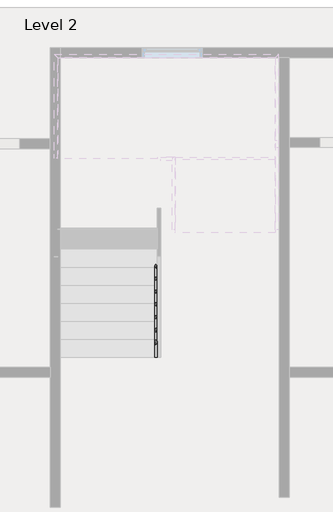
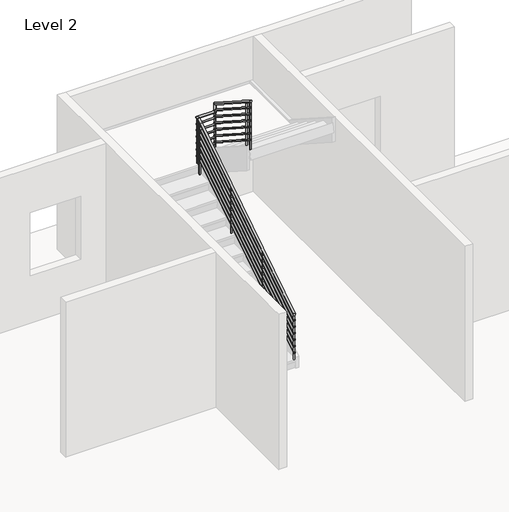
# One storey, part 6 of 7: 1 railing.
"""IFC4 building model written with IfcOpenShell, lengths in millimetres."""

from ifc_helpers import new_model, si_unit, point, frame, frame_2d, origin, place, context, project, spatial, circle_curve, ellipse_curve, trimmed, segment, composite_curve, outline, extrude, element, save
from ifc_brep_helpers import plane_surface, cylinder_surface, advanced_brep

model = new_model("IFC4")

# Units and contexts
model_context = context("Model", 3, world=origin())
ifc_project = project(units=[si_unit("LENGTHUNIT", "METRE", prefix="MILLI")], contexts=[model_context])

# Site, building, storey
site = spatial("IfcSite", under=ifc_project)
building = spatial("IfcBuilding", under=site)
storey = spatial("IfcBuildingStorey", under=building, Name="Level 2", Elevation=3500.0)

# Railing
placement = place(None, origin())
element("IfcRailing", 1, ObjectType="900mm Pipe", at=placement, inside=storey, context=model_context, shape_type="SolidModel", body=[
    advanced_brep(
    [(-504.8393676, 4284.7509075, 4552.7068065), (-544.8393676, 4284.7509075, 4552.7068065), (-504.8393676, 7315.616134, 6497.6470588), (-544.8393676, 7315.616134, 6497.6470588), (-504.8393676, 7337.8781803, 6497.6470588), (-544.8393676, 7377.8781803, 6497.6470588), (-201.3120949, 7337.8781803, 6497.6470588), (-201.3120949, 7377.8781803, 6497.6470588)],
    [
        (0, 1, ellipse_curve(frame((-524.8393676, 4284.7509075, 4552.7068065), z_axis=(0.0, -1.0, 0.0), x_axis=(0.0, 0.0, -1.0)), 23.7637817, 20.0)),
        (1, 0, ellipse_curve(frame((-524.8393676, 4284.7509075, 4552.7068065), z_axis=(0.0, -1.0, 0.0), x_axis=(0.0, 0.0, -1.0)), 23.7637817, 20.0)),
        (0, 2),
        (2, 3, ellipse_curve(frame((-524.8393676, 7315.616134, 6497.6470588), z_axis=(0.0, -0.9595876426002529, -0.2814099432658509), x_axis=(0.0, 0.2814099432658507, -0.9595876426002528)), 20.8422859, 20.0)),
        (3, 1),
        (3, 2, ellipse_curve(frame((-524.8393676, 7315.616134, 6497.6470588), z_axis=(0.0, -0.9595876426002529, -0.2814099432658509), x_axis=(0.0, 0.2814099432658507, -0.9595876426002528)), 20.8422859, 20.0)),
        (2, 4),
        (4, 5, ellipse_curve(frame((-524.8393676, 7357.8781803, 6497.6470588), z_axis=(-0.7071067811865475, -0.7071067811865475, 0.0), x_axis=(0.7071067811865474, -0.7071067811865476, 0.0)), 28.2842712, 20.0)),
        (5, 3),
        (5, 4, ellipse_curve(frame((-524.8393676, 7357.8781803, 6497.6470588), z_axis=(-0.7071067811865475, -0.7071067811865475, 0.0), x_axis=(0.7071067811865474, -0.7071067811865476, 0.0)), 28.2842712, 20.0)),
        (6, 7, ellipse_curve(frame((-201.3120949, 7357.8781803, 6497.6470588), z_axis=(0.7071067811865476, 0.0, 0.7071067811865476), x_axis=(-0.7071067811865474, 0.0, 0.7071067811865476)), 28.2842712, 20.0)),
        (7, 6, ellipse_curve(frame((-201.3120949, 7357.8781803, 6497.6470588), z_axis=(0.7071067811865476, 0.0, 0.7071067811865476), x_axis=(-0.7071067811865474, 0.0, 0.7071067811865476)), 28.2842712, 20.0)),
        (4, 6),
        (7, 5),
    ],
    [
        plane_surface(frame((-524.8393676, 4284.7509075, 4576.4705882), z_axis=(0.0, -1.0, 0.0), x_axis=(0.0, 0.0, 1.0))),
        cylinder_surface(frame((-524.8393676, 4295.5524077, 4559.6382505), z_axis=(0.0, -0.8416168876622212, -0.5400750081254976), x_axis=(-1.0, 0.0, 0.0)), 20.0),
        cylinder_surface(frame((-524.8393676, 7309.7509075, 6497.6470588), z_axis=(0.0, -1.0, 0.0), x_axis=(-1.0, 0.0, 0.0)), 20.0),
        plane_surface(frame((-221.3120949, 7357.8781803, 6517.6470588), z_axis=(0.7071067811865476, 0.0, 0.7071067811865476), x_axis=(0.7071067811865476, 0.0, -0.7071067811865476))),
        cylinder_surface(frame((-524.8393676, 7357.8781803, 6497.6470588), z_axis=(-1.0, 0.0, 0.0), x_axis=(0.0, 1.0, 0.0)), 20.0),
    ],
    [
        (0, [[1, 2]]),
        (1, [[-1, 3, 4, 5]]),
        (1, [[-2, -5, 6, -3]]),
        (2, [[-4, 7, 8, 9]]),
        (2, [[-6, -9, 10, -7]]),
        (3, [[11, 12]]),
        (4, [[-8, 13, -12, 14]]),
        (4, [[-10, -14, -11, -13]]),
    ],
),
    advanced_brep(
    [(-201.3120949, 7337.8781803, 6497.6470588), (-201.3120949, 7377.8781803, 6497.6470588), (-201.3120949, 7337.8781803, 6643.124843), (-201.3120949, 7377.8781803, 6664.9839572)],
    [
        (0, 1, ellipse_curve(frame((-201.3120949, 7357.8781803, 6497.6470588), z_axis=(-0.7071067811865476, 0.0, -0.7071067811865476), x_axis=(0.7071067811865476, 0.0, -0.7071067811865474)), 28.2842712, 20.0)),
        (1, 0, ellipse_curve(frame((-201.3120949, 7357.8781803, 6497.6470588), z_axis=(-0.7071067811865476, 0.0, -0.7071067811865476), x_axis=(0.7071067811865476, 0.0, -0.7071067811865474)), 28.2842712, 20.0)),
        (2, 3, ellipse_curve(frame((-201.3120949, 7357.8781803, 6654.0544001), z_axis=(0.0, -0.47954405004884676, 0.877517808402057), x_axis=(0.0, -0.8775178084020571, -0.47954405004884676)), 22.7915602, 20.0)),
        (3, 2, ellipse_curve(frame((-201.3120949, 7357.8781803, 6654.0544001), z_axis=(0.0, -0.47954405004884676, 0.877517808402057), x_axis=(0.0, -0.8775178084020571, -0.47954405004884676)), 22.7915602, 20.0)),
        (0, 2),
        (3, 1),
    ],
    [
        plane_surface(frame((-201.3120949, 7357.8781803, 6497.6470588), z_axis=(-0.7071067811865476, 0.0, -0.7071067811865476), x_axis=(0.7071067811865476, 0.0, -0.7071067811865476))),
        plane_surface(frame((-201.3120949, 7357.8781803, 6654.0544001), z_axis=(0.0, -0.47954405004884676, 0.877517808402057), x_axis=(1.0, 0.0, 0.0))),
        cylinder_surface(frame((-201.3120949, 7357.8781803, 6497.6470588), z_axis=(0.0, 0.0, -1.0), x_axis=(0.0, 1.0, 0.0)), 20.0),
    ],
    [
        (0, [[1, 2]]),
        (1, [[3, 4]]),
        (2, [[-1, 5, -4, 6]]),
        (2, [[-2, -6, -3, -5]]),
    ],
),
    advanced_brep(
    [(-221.3120949, 7357.8781803, 6654.0544001), (-181.3120949, 7357.8781803, 6654.0544001), (-221.3120949, 6232.4781803, 7376.2362183), (-181.3120949, 6232.4781803, 7376.2362183)],
    [
        (0, 1, ellipse_curve(frame((-201.3120949, 7357.8781803, 6654.0544001), z_axis=(0.0, 0.47954405004884676, -0.877517808402057), x_axis=(0.0, 0.8775178084020568, 0.47954405004884676)), 22.7915602, 20.0)),
        (1, 0, ellipse_curve(frame((-201.3120949, 7357.8781803, 6654.0544001), z_axis=(0.0, 0.47954405004884676, -0.877517808402057), x_axis=(0.0, 0.8775178084020568, 0.47954405004884676)), 22.7915602, 20.0)),
        (2, 3, ellipse_curve(frame((-201.3120949, 6232.4781803, 7376.2362183), z_axis=(0.0, -1.0, 0.0), x_axis=(0.0, 0.0, -1.0)), 23.7637817, 20.0)),
        (3, 2, ellipse_curve(frame((-201.3120949, 6232.4781803, 7376.2362183), z_axis=(0.0, -1.0, 0.0), x_axis=(0.0, 0.0, -1.0)), 23.7637817, 20.0)),
        (0, 2),
        (3, 1),
    ],
    [
        plane_surface(frame((-201.3120949, 7377.8781803, 6664.9839572), z_axis=(0.0, 0.47954405004884676, -0.877517808402057), x_axis=(1.0, 0.0, 0.0))),
        plane_surface(frame((-201.3120949, 6232.4781803, 7400.0), z_axis=(0.0, -1.0, 0.0), x_axis=(0.0, 0.0, -1.0))),
        cylinder_surface(frame((-201.3120949, 7367.0766801, 6648.1516195), z_axis=(0.0, 0.8416168876622208, -0.5400750081254984), x_axis=(1.0, 0.0, 0.0)), 20.0),
    ],
    [
        (0, [[1, 2]]),
        (1, [[3, 4]]),
        (2, [[-1, 5, -4, 6]]),
        (2, [[-2, -6, -3, -5]]),
    ],
),
    advanced_brep(
    [(-539.8393676, 4284.7509075, 4433.647752), (-509.8393676, 4284.7509075, 4433.647752), (-539.8393676, 7309.7509075, 6374.8242225), (-509.8393676, 7309.7509075, 6374.8242225)],
    [
        (0, 1, ellipse_curve(frame((-524.8393676, 4284.7509075, 4433.647752), z_axis=(0.0, -1.0, 0.0), x_axis=(0.0, 0.0, -1.0)), 17.8228363, 15.0)),
        (1, 0, ellipse_curve(frame((-524.8393676, 4284.7509075, 4433.647752), z_axis=(0.0, -1.0, 0.0), x_axis=(0.0, 0.0, -1.0)), 17.8228363, 15.0)),
        (2, 3, ellipse_curve(frame((-524.8393676, 7309.7509075, 6374.8242225), z_axis=(0.0, 1.0, 0.0), x_axis=(0.0, 0.0, -1.0)), 17.8228363, 15.0)),
        (3, 2, ellipse_curve(frame((-524.8393676, 7309.7509075, 6374.8242225), z_axis=(0.0, 1.0, 0.0), x_axis=(0.0, 0.0, -1.0)), 17.8228363, 15.0)),
        (0, 2),
        (3, 1),
    ],
    [
        plane_surface(frame((-524.8393676, 4284.7509075, 4451.4705882), z_axis=(0.0, -1.0, 0.0), x_axis=(0.0, 0.0, 1.0))),
        plane_surface(frame((-524.8393676, 7309.7509075, 6392.6470588), z_axis=(0.0, 1.0, 0.0), x_axis=(0.0, 0.0, 1.0))),
        cylinder_surface(frame((-524.8393676, 4292.8520327, 4438.8463349), z_axis=(0.0, -0.8416168876622212, -0.5400750081254976), x_axis=(1.0, 0.0, 0.0)), 15.0),
    ],
    [
        (0, [[1, 2]]),
        (1, [[3, 4]]),
        (2, [[-1, 5, -4, 6]]),
        (2, [[-2, -6, -3, -5]]),
    ],
),
    advanced_brep(
    [(-539.8393676, 7309.7509075, 6377.6470588), (-509.8393676, 7309.7509075, 6377.6470588), (-539.8393676, 7342.8781803, 6377.6470588), (-509.8393676, 7342.8781803, 6377.6470588)],
    [
        (0, 1, circle_curve(frame((-524.8393676, 7309.7509075, 6377.6470588), z_axis=(0.0, -1.0, 0.0), x_axis=(1.0, 0.0, 0.0)), 15.0)),
        (1, 0, circle_curve(frame((-524.8393676, 7309.7509075, 6377.6470588), z_axis=(0.0, -1.0, 0.0), x_axis=(1.0, 0.0, 0.0)), 15.0)),
        (2, 3, circle_curve(frame((-524.8393676, 7342.8781803, 6377.6470588), z_axis=(0.0, 1.0, 0.0), x_axis=(1.0, 0.0, 0.0)), 15.0)),
        (3, 2, circle_curve(frame((-524.8393676, 7342.8781803, 6377.6470588), z_axis=(0.0, 1.0, 0.0), x_axis=(1.0, 0.0, 0.0)), 15.0)),
        (0, 2),
        (3, 1),
    ],
    [
        plane_surface(frame((-524.8393676, 7309.7509075, 6392.6470588), z_axis=(0.0, -1.0, 0.0), x_axis=(0.0, 0.0, 1.0))),
        plane_surface(frame((-524.8393676, 7342.8781803, 6392.6470588), z_axis=(0.0, 1.0, 0.0), x_axis=(0.0, 0.0, 1.0))),
        cylinder_surface(frame((-524.8393676, 7309.7509075, 6377.6470588), z_axis=(0.0, -1.0, 0.0), x_axis=(1.0, 0.0, 0.0)), 15.0),
    ],
    [
        (0, [[1, 2]]),
        (1, [[3, 4]]),
        (2, [[-1, 5, -4, 6]]),
        (2, [[-2, -6, -3, -5]]),
    ],
),
    advanced_brep(
    [(-539.8393676, 7372.8781803, 6377.6470588), (-539.8393676, 7342.8781803, 6377.6470588), (-216.3120949, 7372.8781803, 6377.6470588), (-216.3120949, 7342.8781803, 6377.6470588)],
    [
        (0, 1, circle_curve(frame((-539.8393676, 7357.8781803, 6377.6470588), z_axis=(-1.0, 0.0, 0.0), x_axis=(0.0, -1.0, 0.0)), 15.0)),
        (1, 0, circle_curve(frame((-539.8393676, 7357.8781803, 6377.6470588), z_axis=(-1.0, 0.0, 0.0), x_axis=(0.0, -1.0, 0.0)), 15.0)),
        (2, 3, circle_curve(frame((-216.3120949, 7357.8781803, 6377.6470588), z_axis=(1.0, 0.0, 0.0), x_axis=(0.0, -1.0, 0.0)), 15.0)),
        (3, 2, circle_curve(frame((-216.3120949, 7357.8781803, 6377.6470588), z_axis=(1.0, 0.0, 0.0), x_axis=(0.0, -1.0, 0.0)), 15.0)),
        (0, 2),
        (3, 1),
    ],
    [
        plane_surface(frame((-539.8393676, 7357.8781803, 6392.6470588), z_axis=(-1.0, 0.0, 0.0), x_axis=(0.0, 1.0, 0.0))),
        plane_surface(frame((-216.3120949, 7357.8781803, 6392.6470588), z_axis=(1.0, 0.0, 0.0), x_axis=(0.0, 1.0, 0.0))),
        cylinder_surface(frame((-539.8393676, 7357.8781803, 6377.6470588), z_axis=(-1.0, 0.0, 0.0), x_axis=(0.0, -1.0, 0.0)), 15.0),
    ],
    [
        (0, [[1, 2]]),
        (1, [[3, 4]]),
        (2, [[-1, 5, -4, 6]]),
        (2, [[-2, -6, -3, -5]]),
    ],
),
    advanced_brep(
    [(-186.3120949, 7372.8781803, 6525.3696771), (-216.3120949, 7372.8781803, 6525.3696771), (-186.3120949, 6232.4781803, 7257.1771637), (-216.3120949, 6232.4781803, 7257.1771637)],
    [
        (0, 1, ellipse_curve(frame((-201.3120949, 7372.8781803, 6525.3696771), z_axis=(0.0, 1.0, 0.0), x_axis=(0.0, 0.0, -1.0)), 17.8228363, 15.0)),
        (1, 0, ellipse_curve(frame((-201.3120949, 7372.8781803, 6525.3696771), z_axis=(0.0, 1.0, 0.0), x_axis=(0.0, 0.0, -1.0)), 17.8228363, 15.0)),
        (2, 3, ellipse_curve(frame((-201.3120949, 6232.4781803, 7257.1771637), z_axis=(0.0, -1.0, 0.0), x_axis=(0.0, 0.0, -1.0)), 17.8228363, 15.0)),
        (3, 2, ellipse_curve(frame((-201.3120949, 6232.4781803, 7257.1771637), z_axis=(0.0, -1.0, 0.0), x_axis=(0.0, 0.0, -1.0)), 17.8228363, 15.0)),
        (0, 2),
        (3, 1),
    ],
    [
        plane_surface(frame((-201.3120949, 7372.8781803, 6543.1925134), z_axis=(0.0, 1.0, 0.0), x_axis=(0.0, 0.0, -1.0))),
        plane_surface(frame((-201.3120949, 6232.4781803, 7275.0), z_axis=(0.0, -1.0, 0.0), x_axis=(0.0, 0.0, -1.0))),
        cylinder_surface(frame((-201.3120949, 7364.7770552, 6530.5682601), z_axis=(0.0, 0.8416168876622208, -0.5400750081254984), x_axis=(-1.0, 0.0, 0.0)), 15.0),
    ],
    [
        (0, [[1, 2]]),
        (1, [[3, 4]]),
        (2, [[-1, 5, -4, 6]]),
        (2, [[-2, -6, -3, -5]]),
    ],
),
    advanced_brep(
    [(-539.8393676, 4284.7509075, 4308.647752), (-509.8393676, 4284.7509075, 4308.647752), (-539.8393676, 7309.7509075, 6249.8242225), (-509.8393676, 7309.7509075, 6249.8242225)],
    [
        (0, 1, ellipse_curve(frame((-524.8393676, 4284.7509075, 4308.647752), z_axis=(0.0, -1.0, 0.0), x_axis=(0.0, 0.0, -1.0)), 17.8228363, 15.0)),
        (1, 0, ellipse_curve(frame((-524.8393676, 4284.7509075, 4308.647752), z_axis=(0.0, -1.0, 0.0), x_axis=(0.0, 0.0, -1.0)), 17.8228363, 15.0)),
        (2, 3, ellipse_curve(frame((-524.8393676, 7309.7509075, 6249.8242225), z_axis=(0.0, 1.0, 0.0), x_axis=(0.0, 0.0, -1.0)), 17.8228363, 15.0)),
        (3, 2, ellipse_curve(frame((-524.8393676, 7309.7509075, 6249.8242225), z_axis=(0.0, 1.0, 0.0), x_axis=(0.0, 0.0, -1.0)), 17.8228363, 15.0)),
        (0, 2),
        (3, 1),
    ],
    [
        plane_surface(frame((-524.8393676, 4284.7509075, 4326.4705882), z_axis=(0.0, -1.0, 0.0), x_axis=(0.0, 0.0, 1.0))),
        plane_surface(frame((-524.8393676, 7309.7509075, 6267.6470588), z_axis=(0.0, 1.0, 0.0), x_axis=(0.0, 0.0, 1.0))),
        cylinder_surface(frame((-524.8393676, 4292.8520327, 4313.8463349), z_axis=(0.0, -0.8416168876622212, -0.5400750081254976), x_axis=(1.0, 0.0, 0.0)), 15.0),
    ],
    [
        (0, [[1, 2]]),
        (1, [[3, 4]]),
        (2, [[-1, 5, -4, 6]]),
        (2, [[-2, -6, -3, -5]]),
    ],
),
    advanced_brep(
    [(-539.8393676, 7309.7509075, 6252.6470588), (-509.8393676, 7309.7509075, 6252.6470588), (-539.8393676, 7342.8781803, 6252.6470588), (-509.8393676, 7342.8781803, 6252.6470588)],
    [
        (0, 1, circle_curve(frame((-524.8393676, 7309.7509075, 6252.6470588), z_axis=(0.0, -1.0, 0.0), x_axis=(1.0, 0.0, 0.0)), 15.0)),
        (1, 0, circle_curve(frame((-524.8393676, 7309.7509075, 6252.6470588), z_axis=(0.0, -1.0, 0.0), x_axis=(1.0, 0.0, 0.0)), 15.0)),
        (2, 3, circle_curve(frame((-524.8393676, 7342.8781803, 6252.6470588), z_axis=(0.0, 1.0, 0.0), x_axis=(1.0, 0.0, 0.0)), 15.0)),
        (3, 2, circle_curve(frame((-524.8393676, 7342.8781803, 6252.6470588), z_axis=(0.0, 1.0, 0.0), x_axis=(1.0, 0.0, 0.0)), 15.0)),
        (0, 2),
        (3, 1),
    ],
    [
        plane_surface(frame((-524.8393676, 7309.7509075, 6267.6470588), z_axis=(0.0, -1.0, 0.0), x_axis=(0.0, 0.0, 1.0))),
        plane_surface(frame((-524.8393676, 7342.8781803, 6267.6470588), z_axis=(0.0, 1.0, 0.0), x_axis=(0.0, 0.0, 1.0))),
        cylinder_surface(frame((-524.8393676, 7309.7509075, 6252.6470588), z_axis=(0.0, -1.0, 0.0), x_axis=(1.0, 0.0, 0.0)), 15.0),
    ],
    [
        (0, [[1, 2]]),
        (1, [[3, 4]]),
        (2, [[-1, 5, -4, 6]]),
        (2, [[-2, -6, -3, -5]]),
    ],
),
    advanced_brep(
    [(-539.8393676, 7372.8781803, 6252.6470588), (-539.8393676, 7342.8781803, 6252.6470588), (-216.3120949, 7372.8781803, 6252.6470588), (-216.3120949, 7342.8781803, 6252.6470588)],
    [
        (0, 1, circle_curve(frame((-539.8393676, 7357.8781803, 6252.6470588), z_axis=(-1.0, 0.0, 0.0), x_axis=(0.0, -1.0, 0.0)), 15.0)),
        (1, 0, circle_curve(frame((-539.8393676, 7357.8781803, 6252.6470588), z_axis=(-1.0, 0.0, 0.0), x_axis=(0.0, -1.0, 0.0)), 15.0)),
        (2, 3, circle_curve(frame((-216.3120949, 7357.8781803, 6252.6470588), z_axis=(1.0, 0.0, 0.0), x_axis=(0.0, -1.0, 0.0)), 15.0)),
        (3, 2, circle_curve(frame((-216.3120949, 7357.8781803, 6252.6470588), z_axis=(1.0, 0.0, 0.0), x_axis=(0.0, -1.0, 0.0)), 15.0)),
        (0, 2),
        (3, 1),
    ],
    [
        plane_surface(frame((-539.8393676, 7357.8781803, 6267.6470588), z_axis=(-1.0, 0.0, 0.0), x_axis=(0.0, 1.0, 0.0))),
        plane_surface(frame((-216.3120949, 7357.8781803, 6267.6470588), z_axis=(1.0, 0.0, 0.0), x_axis=(0.0, 1.0, 0.0))),
        cylinder_surface(frame((-539.8393676, 7357.8781803, 6252.6470588), z_axis=(-1.0, 0.0, 0.0), x_axis=(0.0, -1.0, 0.0)), 15.0),
    ],
    [
        (0, [[1, 2]]),
        (1, [[3, 4]]),
        (2, [[-1, 5, -4, 6]]),
        (2, [[-2, -6, -3, -5]]),
    ],
),
    advanced_brep(
    [(-186.3120949, 7372.8781803, 6400.3696771), (-216.3120949, 7372.8781803, 6400.3696771), (-186.3120949, 6232.4781803, 7132.1771637), (-216.3120949, 6232.4781803, 7132.1771637)],
    [
        (0, 1, ellipse_curve(frame((-201.3120949, 7372.8781803, 6400.3696771), z_axis=(0.0, 1.0, 0.0), x_axis=(0.0, 0.0, -1.0)), 17.8228363, 15.0)),
        (1, 0, ellipse_curve(frame((-201.3120949, 7372.8781803, 6400.3696771), z_axis=(0.0, 1.0, 0.0), x_axis=(0.0, 0.0, -1.0)), 17.8228363, 15.0)),
        (2, 3, ellipse_curve(frame((-201.3120949, 6232.4781803, 7132.1771637), z_axis=(0.0, -1.0, 0.0), x_axis=(0.0, 0.0, -1.0)), 17.8228363, 15.0)),
        (3, 2, ellipse_curve(frame((-201.3120949, 6232.4781803, 7132.1771637), z_axis=(0.0, -1.0, 0.0), x_axis=(0.0, 0.0, -1.0)), 17.8228363, 15.0)),
        (0, 2),
        (3, 1),
    ],
    [
        plane_surface(frame((-201.3120949, 7372.8781803, 6418.1925134), z_axis=(0.0, 1.0, 0.0), x_axis=(0.0, 0.0, -1.0))),
        plane_surface(frame((-201.3120949, 6232.4781803, 7150.0), z_axis=(0.0, -1.0, 0.0), x_axis=(0.0, 0.0, -1.0))),
        cylinder_surface(frame((-201.3120949, 7364.7770552, 6405.5682601), z_axis=(0.0, 0.8416168876622208, -0.5400750081254984), x_axis=(-1.0, 0.0, 0.0)), 15.0),
    ],
    [
        (0, [[1, 2]]),
        (1, [[3, 4]]),
        (2, [[-1, 5, -4, 6]]),
        (2, [[-2, -6, -3, -5]]),
    ],
),
    advanced_brep(
    [(-539.8393676, 4284.7509075, 4183.647752), (-509.8393676, 4284.7509075, 4183.647752), (-539.8393676, 7309.7509075, 6124.8242225), (-509.8393676, 7309.7509075, 6124.8242225)],
    [
        (0, 1, ellipse_curve(frame((-524.8393676, 4284.7509075, 4183.647752), z_axis=(0.0, -1.0, 0.0), x_axis=(0.0, 0.0, -1.0)), 17.8228363, 15.0)),
        (1, 0, ellipse_curve(frame((-524.8393676, 4284.7509075, 4183.647752), z_axis=(0.0, -1.0, 0.0), x_axis=(0.0, 0.0, -1.0)), 17.8228363, 15.0)),
        (2, 3, ellipse_curve(frame((-524.8393676, 7309.7509075, 6124.8242225), z_axis=(0.0, 1.0, 0.0), x_axis=(0.0, 0.0, -1.0)), 17.8228363, 15.0)),
        (3, 2, ellipse_curve(frame((-524.8393676, 7309.7509075, 6124.8242225), z_axis=(0.0, 1.0, 0.0), x_axis=(0.0, 0.0, -1.0)), 17.8228363, 15.0)),
        (0, 2),
        (3, 1),
    ],
    [
        plane_surface(frame((-524.8393676, 4284.7509075, 4201.4705882), z_axis=(0.0, -1.0, 0.0), x_axis=(0.0, 0.0, 1.0))),
        plane_surface(frame((-524.8393676, 7309.7509075, 6142.6470588), z_axis=(0.0, 1.0, 0.0), x_axis=(0.0, 0.0, 1.0))),
        cylinder_surface(frame((-524.8393676, 4292.8520327, 4188.8463349), z_axis=(0.0, -0.8416168876622212, -0.5400750081254976), x_axis=(1.0, 0.0, 0.0)), 15.0),
    ],
    [
        (0, [[1, 2]]),
        (1, [[3, 4]]),
        (2, [[-1, 5, -4, 6]]),
        (2, [[-2, -6, -3, -5]]),
    ],
),
    advanced_brep(
    [(-539.8393676, 7309.7509075, 6127.6470588), (-509.8393676, 7309.7509075, 6127.6470588), (-539.8393676, 7342.8781803, 6127.6470588), (-509.8393676, 7342.8781803, 6127.6470588)],
    [
        (0, 1, circle_curve(frame((-524.8393676, 7309.7509075, 6127.6470588), z_axis=(0.0, -1.0, 0.0), x_axis=(1.0, 0.0, 0.0)), 15.0)),
        (1, 0, circle_curve(frame((-524.8393676, 7309.7509075, 6127.6470588), z_axis=(0.0, -1.0, 0.0), x_axis=(1.0, 0.0, 0.0)), 15.0)),
        (2, 3, circle_curve(frame((-524.8393676, 7342.8781803, 6127.6470588), z_axis=(0.0, 1.0, 0.0), x_axis=(1.0, 0.0, 0.0)), 15.0)),
        (3, 2, circle_curve(frame((-524.8393676, 7342.8781803, 6127.6470588), z_axis=(0.0, 1.0, 0.0), x_axis=(1.0, 0.0, 0.0)), 15.0)),
        (0, 2),
        (3, 1),
    ],
    [
        plane_surface(frame((-524.8393676, 7309.7509075, 6142.6470588), z_axis=(0.0, -1.0, 0.0), x_axis=(0.0, 0.0, 1.0))),
        plane_surface(frame((-524.8393676, 7342.8781803, 6142.6470588), z_axis=(0.0, 1.0, 0.0), x_axis=(0.0, 0.0, 1.0))),
        cylinder_surface(frame((-524.8393676, 7309.7509075, 6127.6470588), z_axis=(0.0, -1.0, 0.0), x_axis=(1.0, 0.0, 0.0)), 15.0),
    ],
    [
        (0, [[1, 2]]),
        (1, [[3, 4]]),
        (2, [[-1, 5, -4, 6]]),
        (2, [[-2, -6, -3, -5]]),
    ],
),
    advanced_brep(
    [(-539.8393676, 7372.8781803, 6127.6470588), (-539.8393676, 7342.8781803, 6127.6470588), (-216.3120949, 7372.8781803, 6127.6470588), (-216.3120949, 7342.8781803, 6127.6470588)],
    [
        (0, 1, circle_curve(frame((-539.8393676, 7357.8781803, 6127.6470588), z_axis=(-1.0, 0.0, 0.0), x_axis=(0.0, -1.0, 0.0)), 15.0)),
        (1, 0, circle_curve(frame((-539.8393676, 7357.8781803, 6127.6470588), z_axis=(-1.0, 0.0, 0.0), x_axis=(0.0, -1.0, 0.0)), 15.0)),
        (2, 3, circle_curve(frame((-216.3120949, 7357.8781803, 6127.6470588), z_axis=(1.0, 0.0, 0.0), x_axis=(0.0, -1.0, 0.0)), 15.0)),
        (3, 2, circle_curve(frame((-216.3120949, 7357.8781803, 6127.6470588), z_axis=(1.0, 0.0, 0.0), x_axis=(0.0, -1.0, 0.0)), 15.0)),
        (0, 2),
        (3, 1),
    ],
    [
        plane_surface(frame((-539.8393676, 7357.8781803, 6142.6470588), z_axis=(-1.0, 0.0, 0.0), x_axis=(0.0, 1.0, 0.0))),
        plane_surface(frame((-216.3120949, 7357.8781803, 6142.6470588), z_axis=(1.0, 0.0, 0.0), x_axis=(0.0, 1.0, 0.0))),
        cylinder_surface(frame((-539.8393676, 7357.8781803, 6127.6470588), z_axis=(-1.0, 0.0, 0.0), x_axis=(0.0, -1.0, 0.0)), 15.0),
    ],
    [
        (0, [[1, 2]]),
        (1, [[3, 4]]),
        (2, [[-1, 5, -4, 6]]),
        (2, [[-2, -6, -3, -5]]),
    ],
),
    advanced_brep(
    [(-186.3120949, 7372.8781803, 6275.3696771), (-216.3120949, 7372.8781803, 6275.3696771), (-186.3120949, 6232.4781803, 7007.1771637), (-216.3120949, 6232.4781803, 7007.1771637)],
    [
        (0, 1, ellipse_curve(frame((-201.3120949, 7372.8781803, 6275.3696771), z_axis=(0.0, 1.0, 0.0), x_axis=(0.0, 0.0, -1.0)), 17.8228363, 15.0)),
        (1, 0, ellipse_curve(frame((-201.3120949, 7372.8781803, 6275.3696771), z_axis=(0.0, 1.0, 0.0), x_axis=(0.0, 0.0, -1.0)), 17.8228363, 15.0)),
        (2, 3, ellipse_curve(frame((-201.3120949, 6232.4781803, 7007.1771637), z_axis=(0.0, -1.0, 0.0), x_axis=(0.0, 0.0, -1.0)), 17.8228363, 15.0)),
        (3, 2, ellipse_curve(frame((-201.3120949, 6232.4781803, 7007.1771637), z_axis=(0.0, -1.0, 0.0), x_axis=(0.0, 0.0, -1.0)), 17.8228363, 15.0)),
        (0, 2),
        (3, 1),
    ],
    [
        plane_surface(frame((-201.3120949, 7372.8781803, 6293.1925134), z_axis=(0.0, 1.0, 0.0), x_axis=(0.0, 0.0, -1.0))),
        plane_surface(frame((-201.3120949, 6232.4781803, 7025.0), z_axis=(0.0, -1.0, 0.0), x_axis=(0.0, 0.0, -1.0))),
        cylinder_surface(frame((-201.3120949, 7364.7770552, 6280.5682601), z_axis=(0.0, 0.8416168876622208, -0.5400750081254984), x_axis=(-1.0, 0.0, 0.0)), 15.0),
    ],
    [
        (0, [[1, 2]]),
        (1, [[3, 4]]),
        (2, [[-1, 5, -4, 6]]),
        (2, [[-2, -6, -3, -5]]),
    ],
),
    advanced_brep(
    [(-539.8393676, 4284.7509075, 4058.647752), (-509.8393676, 4284.7509075, 4058.647752), (-539.8393676, 7309.7509075, 5999.8242225), (-509.8393676, 7309.7509075, 5999.8242225)],
    [
        (0, 1, ellipse_curve(frame((-524.8393676, 4284.7509075, 4058.647752), z_axis=(0.0, -1.0, 0.0), x_axis=(0.0, 0.0, -1.0)), 17.8228363, 15.0)),
        (1, 0, ellipse_curve(frame((-524.8393676, 4284.7509075, 4058.647752), z_axis=(0.0, -1.0, 0.0), x_axis=(0.0, 0.0, -1.0)), 17.8228363, 15.0)),
        (2, 3, ellipse_curve(frame((-524.8393676, 7309.7509075, 5999.8242225), z_axis=(0.0, 1.0, 0.0), x_axis=(0.0, 0.0, -1.0)), 17.8228363, 15.0)),
        (3, 2, ellipse_curve(frame((-524.8393676, 7309.7509075, 5999.8242225), z_axis=(0.0, 1.0, 0.0), x_axis=(0.0, 0.0, -1.0)), 17.8228363, 15.0)),
        (0, 2),
        (3, 1),
    ],
    [
        plane_surface(frame((-524.8393676, 4284.7509075, 4076.4705882), z_axis=(0.0, -1.0, 0.0), x_axis=(0.0, 0.0, 1.0))),
        plane_surface(frame((-524.8393676, 7309.7509075, 6017.6470588), z_axis=(0.0, 1.0, 0.0), x_axis=(0.0, 0.0, 1.0))),
        cylinder_surface(frame((-524.8393676, 4292.8520327, 4063.8463349), z_axis=(0.0, -0.8416168876622212, -0.5400750081254976), x_axis=(1.0, 0.0, 0.0)), 15.0),
    ],
    [
        (0, [[1, 2]]),
        (1, [[3, 4]]),
        (2, [[-1, 5, -4, 6]]),
        (2, [[-2, -6, -3, -5]]),
    ],
),
    advanced_brep(
    [(-539.8393676, 7309.7509075, 6002.6470588), (-509.8393676, 7309.7509075, 6002.6470588), (-539.8393676, 7342.8781803, 6002.6470588), (-509.8393676, 7342.8781803, 6002.6470588)],
    [
        (0, 1, circle_curve(frame((-524.8393676, 7309.7509075, 6002.6470588), z_axis=(0.0, -1.0, 0.0), x_axis=(1.0, 0.0, 0.0)), 15.0)),
        (1, 0, circle_curve(frame((-524.8393676, 7309.7509075, 6002.6470588), z_axis=(0.0, -1.0, 0.0), x_axis=(1.0, 0.0, 0.0)), 15.0)),
        (2, 3, circle_curve(frame((-524.8393676, 7342.8781803, 6002.6470588), z_axis=(0.0, 1.0, 0.0), x_axis=(1.0, 0.0, 0.0)), 15.0)),
        (3, 2, circle_curve(frame((-524.8393676, 7342.8781803, 6002.6470588), z_axis=(0.0, 1.0, 0.0), x_axis=(1.0, 0.0, 0.0)), 15.0)),
        (0, 2),
        (3, 1),
    ],
    [
        plane_surface(frame((-524.8393676, 7309.7509075, 6017.6470588), z_axis=(0.0, -1.0, 0.0), x_axis=(0.0, 0.0, 1.0))),
        plane_surface(frame((-524.8393676, 7342.8781803, 6017.6470588), z_axis=(0.0, 1.0, 0.0), x_axis=(0.0, 0.0, 1.0))),
        cylinder_surface(frame((-524.8393676, 7309.7509075, 6002.6470588), z_axis=(0.0, -1.0, 0.0), x_axis=(1.0, 0.0, 0.0)), 15.0),
    ],
    [
        (0, [[1, 2]]),
        (1, [[3, 4]]),
        (2, [[-1, 5, -4, 6]]),
        (2, [[-2, -6, -3, -5]]),
    ],
),
    advanced_brep(
    [(-539.8393676, 7372.8781803, 6002.6470588), (-539.8393676, 7342.8781803, 6002.6470588), (-216.3120949, 7372.8781803, 6002.6470588), (-216.3120949, 7342.8781803, 6002.6470588)],
    [
        (0, 1, circle_curve(frame((-539.8393676, 7357.8781803, 6002.6470588), z_axis=(-1.0, 0.0, 0.0), x_axis=(0.0, -1.0, 0.0)), 15.0)),
        (1, 0, circle_curve(frame((-539.8393676, 7357.8781803, 6002.6470588), z_axis=(-1.0, 0.0, 0.0), x_axis=(0.0, -1.0, 0.0)), 15.0)),
        (2, 3, circle_curve(frame((-216.3120949, 7357.8781803, 6002.6470588), z_axis=(1.0, 0.0, 0.0), x_axis=(0.0, -1.0, 0.0)), 15.0)),
        (3, 2, circle_curve(frame((-216.3120949, 7357.8781803, 6002.6470588), z_axis=(1.0, 0.0, 0.0), x_axis=(0.0, -1.0, 0.0)), 15.0)),
        (0, 2),
        (3, 1),
    ],
    [
        plane_surface(frame((-539.8393676, 7357.8781803, 6017.6470588), z_axis=(-1.0, 0.0, 0.0), x_axis=(0.0, 1.0, 0.0))),
        plane_surface(frame((-216.3120949, 7357.8781803, 6017.6470588), z_axis=(1.0, 0.0, 0.0), x_axis=(0.0, 1.0, 0.0))),
        cylinder_surface(frame((-539.8393676, 7357.8781803, 6002.6470588), z_axis=(-1.0, 0.0, 0.0), x_axis=(0.0, -1.0, 0.0)), 15.0),
    ],
    [
        (0, [[1, 2]]),
        (1, [[3, 4]]),
        (2, [[-1, 5, -4, 6]]),
        (2, [[-2, -6, -3, -5]]),
    ],
),
    advanced_brep(
    [(-186.3120949, 7372.8781803, 6150.3696771), (-216.3120949, 7372.8781803, 6150.3696771), (-186.3120949, 6232.4781803, 6882.1771637), (-216.3120949, 6232.4781803, 6882.1771637)],
    [
        (0, 1, ellipse_curve(frame((-201.3120949, 7372.8781803, 6150.3696771), z_axis=(0.0, 1.0, 0.0), x_axis=(0.0, 0.0, -1.0)), 17.8228363, 15.0)),
        (1, 0, ellipse_curve(frame((-201.3120949, 7372.8781803, 6150.3696771), z_axis=(0.0, 1.0, 0.0), x_axis=(0.0, 0.0, -1.0)), 17.8228363, 15.0)),
        (2, 3, ellipse_curve(frame((-201.3120949, 6232.4781803, 6882.1771637), z_axis=(0.0, -1.0, 0.0), x_axis=(0.0, 0.0, -1.0)), 17.8228363, 15.0)),
        (3, 2, ellipse_curve(frame((-201.3120949, 6232.4781803, 6882.1771637), z_axis=(0.0, -1.0, 0.0), x_axis=(0.0, 0.0, -1.0)), 17.8228363, 15.0)),
        (0, 2),
        (3, 1),
    ],
    [
        plane_surface(frame((-201.3120949, 7372.8781803, 6168.1925134), z_axis=(0.0, 1.0, 0.0), x_axis=(0.0, 0.0, -1.0))),
        plane_surface(frame((-201.3120949, 6232.4781803, 6900.0), z_axis=(0.0, -1.0, 0.0), x_axis=(0.0, 0.0, -1.0))),
        cylinder_surface(frame((-201.3120949, 7364.7770552, 6155.5682601), z_axis=(0.0, 0.8416168876622208, -0.5400750081254984), x_axis=(-1.0, 0.0, 0.0)), 15.0),
    ],
    [
        (0, [[1, 2]]),
        (1, [[3, 4]]),
        (2, [[-1, 5, -4, 6]]),
        (2, [[-2, -6, -3, -5]]),
    ],
),
    advanced_brep(
    [(-539.8393676, 4284.7509075, 3933.647752), (-509.8393676, 4284.7509075, 3933.647752), (-539.8393676, 7309.7509075, 5874.8242225), (-509.8393676, 7309.7509075, 5874.8242225)],
    [
        (0, 1, ellipse_curve(frame((-524.8393676, 4284.7509075, 3933.647752), z_axis=(0.0, -1.0, 0.0), x_axis=(0.0, 0.0, -1.0)), 17.8228363, 15.0)),
        (1, 0, ellipse_curve(frame((-524.8393676, 4284.7509075, 3933.647752), z_axis=(0.0, -1.0, 0.0), x_axis=(0.0, 0.0, -1.0)), 17.8228363, 15.0)),
        (2, 3, ellipse_curve(frame((-524.8393676, 7309.7509075, 5874.8242225), z_axis=(0.0, 1.0, 0.0), x_axis=(0.0, 0.0, -1.0)), 17.8228363, 15.0)),
        (3, 2, ellipse_curve(frame((-524.8393676, 7309.7509075, 5874.8242225), z_axis=(0.0, 1.0, 0.0), x_axis=(0.0, 0.0, -1.0)), 17.8228363, 15.0)),
        (0, 2),
        (3, 1),
    ],
    [
        plane_surface(frame((-524.8393676, 4284.7509075, 3951.4705882), z_axis=(0.0, -1.0, 0.0), x_axis=(0.0, 0.0, 1.0))),
        plane_surface(frame((-524.8393676, 7309.7509075, 5892.6470588), z_axis=(0.0, 1.0, 0.0), x_axis=(0.0, 0.0, 1.0))),
        cylinder_surface(frame((-524.8393676, 4292.8520327, 3938.8463349), z_axis=(0.0, -0.8416168876622212, -0.5400750081254976), x_axis=(1.0, 0.0, 0.0)), 15.0),
    ],
    [
        (0, [[1, 2]]),
        (1, [[3, 4]]),
        (2, [[-1, 5, -4, 6]]),
        (2, [[-2, -6, -3, -5]]),
    ],
),
    advanced_brep(
    [(-539.8393676, 7309.7509075, 5877.6470588), (-509.8393676, 7309.7509075, 5877.6470588), (-539.8393676, 7342.8781803, 5877.6470588), (-509.8393676, 7342.8781803, 5877.6470588)],
    [
        (0, 1, circle_curve(frame((-524.8393676, 7309.7509075, 5877.6470588), z_axis=(0.0, -1.0, 0.0), x_axis=(1.0, 0.0, 0.0)), 15.0)),
        (1, 0, circle_curve(frame((-524.8393676, 7309.7509075, 5877.6470588), z_axis=(0.0, -1.0, 0.0), x_axis=(1.0, 0.0, 0.0)), 15.0)),
        (2, 3, circle_curve(frame((-524.8393676, 7342.8781803, 5877.6470588), z_axis=(0.0, 1.0, 0.0), x_axis=(1.0, 0.0, 0.0)), 15.0)),
        (3, 2, circle_curve(frame((-524.8393676, 7342.8781803, 5877.6470588), z_axis=(0.0, 1.0, 0.0), x_axis=(1.0, 0.0, 0.0)), 15.0)),
        (0, 2),
        (3, 1),
    ],
    [
        plane_surface(frame((-524.8393676, 7309.7509075, 5892.6470588), z_axis=(0.0, -1.0, 0.0), x_axis=(0.0, 0.0, 1.0))),
        plane_surface(frame((-524.8393676, 7342.8781803, 5892.6470588), z_axis=(0.0, 1.0, 0.0), x_axis=(0.0, 0.0, 1.0))),
        cylinder_surface(frame((-524.8393676, 7309.7509075, 5877.6470588), z_axis=(0.0, -1.0, 0.0), x_axis=(1.0, 0.0, 0.0)), 15.0),
    ],
    [
        (0, [[1, 2]]),
        (1, [[3, 4]]),
        (2, [[-1, 5, -4, 6]]),
        (2, [[-2, -6, -3, -5]]),
    ],
),
    advanced_brep(
    [(-539.8393676, 7372.8781803, 5877.6470588), (-539.8393676, 7342.8781803, 5877.6470588), (-216.3120949, 7372.8781803, 5877.6470588), (-216.3120949, 7342.8781803, 5877.6470588)],
    [
        (0, 1, circle_curve(frame((-539.8393676, 7357.8781803, 5877.6470588), z_axis=(-1.0, 0.0, 0.0), x_axis=(0.0, -1.0, 0.0)), 15.0)),
        (1, 0, circle_curve(frame((-539.8393676, 7357.8781803, 5877.6470588), z_axis=(-1.0, 0.0, 0.0), x_axis=(0.0, -1.0, 0.0)), 15.0)),
        (2, 3, circle_curve(frame((-216.3120949, 7357.8781803, 5877.6470588), z_axis=(1.0, 0.0, 0.0), x_axis=(0.0, -1.0, 0.0)), 15.0)),
        (3, 2, circle_curve(frame((-216.3120949, 7357.8781803, 5877.6470588), z_axis=(1.0, 0.0, 0.0), x_axis=(0.0, -1.0, 0.0)), 15.0)),
        (0, 2),
        (3, 1),
    ],
    [
        plane_surface(frame((-539.8393676, 7357.8781803, 5892.6470588), z_axis=(-1.0, 0.0, 0.0), x_axis=(0.0, 1.0, 0.0))),
        plane_surface(frame((-216.3120949, 7357.8781803, 5892.6470588), z_axis=(1.0, 0.0, 0.0), x_axis=(0.0, 1.0, 0.0))),
        cylinder_surface(frame((-539.8393676, 7357.8781803, 5877.6470588), z_axis=(-1.0, 0.0, 0.0), x_axis=(0.0, -1.0, 0.0)), 15.0),
    ],
    [
        (0, [[1, 2]]),
        (1, [[3, 4]]),
        (2, [[-1, 5, -4, 6]]),
        (2, [[-2, -6, -3, -5]]),
    ],
),
    advanced_brep(
    [(-186.3120949, 7372.8781803, 6025.3696771), (-216.3120949, 7372.8781803, 6025.3696771), (-186.3120949, 6232.4781803, 6757.1771637), (-216.3120949, 6232.4781803, 6757.1771637)],
    [
        (0, 1, ellipse_curve(frame((-201.3120949, 7372.8781803, 6025.3696771), z_axis=(0.0, 1.0, 0.0), x_axis=(0.0, 0.0, -1.0)), 17.8228363, 15.0)),
        (1, 0, ellipse_curve(frame((-201.3120949, 7372.8781803, 6025.3696771), z_axis=(0.0, 1.0, 0.0), x_axis=(0.0, 0.0, -1.0)), 17.8228363, 15.0)),
        (2, 3, ellipse_curve(frame((-201.3120949, 6232.4781803, 6757.1771637), z_axis=(0.0, -1.0, 0.0), x_axis=(0.0, 0.0, -1.0)), 17.8228363, 15.0)),
        (3, 2, ellipse_curve(frame((-201.3120949, 6232.4781803, 6757.1771637), z_axis=(0.0, -1.0, 0.0), x_axis=(0.0, 0.0, -1.0)), 17.8228363, 15.0)),
        (0, 2),
        (3, 1),
    ],
    [
        plane_surface(frame((-201.3120949, 7372.8781803, 6043.1925134), z_axis=(0.0, 1.0, 0.0), x_axis=(0.0, 0.0, -1.0))),
        plane_surface(frame((-201.3120949, 6232.4781803, 6775.0), z_axis=(0.0, -1.0, 0.0), x_axis=(0.0, 0.0, -1.0))),
        cylinder_surface(frame((-201.3120949, 7364.7770552, 6030.5682601), z_axis=(0.0, 0.8416168876622208, -0.5400750081254984), x_axis=(-1.0, 0.0, 0.0)), 15.0),
    ],
    [
        (0, [[1, 2]]),
        (1, [[3, 4]]),
        (2, [[-1, 5, -4, 6]]),
        (2, [[-2, -6, -3, -5]]),
    ],
),
    advanced_brep(
    [(-539.8393676, 4284.7509075, 3808.647752), (-509.8393676, 4284.7509075, 3808.647752), (-539.8393676, 7309.7509075, 5749.8242225), (-509.8393676, 7309.7509075, 5749.8242225)],
    [
        (0, 1, ellipse_curve(frame((-524.8393676, 4284.7509075, 3808.647752), z_axis=(0.0, -1.0, 0.0), x_axis=(0.0, 0.0, -1.0)), 17.8228363, 15.0)),
        (1, 0, ellipse_curve(frame((-524.8393676, 4284.7509075, 3808.647752), z_axis=(0.0, -1.0, 0.0), x_axis=(0.0, 0.0, -1.0)), 17.8228363, 15.0)),
        (2, 3, ellipse_curve(frame((-524.8393676, 7309.7509075, 5749.8242225), z_axis=(0.0, 1.0, 0.0), x_axis=(0.0, 0.0, -1.0)), 17.8228363, 15.0)),
        (3, 2, ellipse_curve(frame((-524.8393676, 7309.7509075, 5749.8242225), z_axis=(0.0, 1.0, 0.0), x_axis=(0.0, 0.0, -1.0)), 17.8228363, 15.0)),
        (0, 2),
        (3, 1),
    ],
    [
        plane_surface(frame((-524.8393676, 4284.7509075, 3826.4705882), z_axis=(0.0, -1.0, 0.0), x_axis=(0.0, 0.0, 1.0))),
        plane_surface(frame((-524.8393676, 7309.7509075, 5767.6470588), z_axis=(0.0, 1.0, 0.0), x_axis=(0.0, 0.0, 1.0))),
        cylinder_surface(frame((-524.8393676, 4292.8520327, 3813.8463349), z_axis=(0.0, -0.8416168876622212, -0.5400750081254976), x_axis=(1.0, 0.0, 0.0)), 15.0),
    ],
    [
        (0, [[1, 2]]),
        (1, [[3, 4]]),
        (2, [[-1, 5, -4, 6]]),
        (2, [[-2, -6, -3, -5]]),
    ],
),
    advanced_brep(
    [(-539.8393676, 7309.7509075, 5752.6470588), (-509.8393676, 7309.7509075, 5752.6470588), (-539.8393676, 7342.8781803, 5752.6470588), (-509.8393676, 7342.8781803, 5752.6470588)],
    [
        (0, 1, circle_curve(frame((-524.8393676, 7309.7509075, 5752.6470588), z_axis=(0.0, -1.0, 0.0), x_axis=(1.0, 0.0, 0.0)), 15.0)),
        (1, 0, circle_curve(frame((-524.8393676, 7309.7509075, 5752.6470588), z_axis=(0.0, -1.0, 0.0), x_axis=(1.0, 0.0, 0.0)), 15.0)),
        (2, 3, circle_curve(frame((-524.8393676, 7342.8781803, 5752.6470588), z_axis=(0.0, 1.0, 0.0), x_axis=(1.0, 0.0, 0.0)), 15.0)),
        (3, 2, circle_curve(frame((-524.8393676, 7342.8781803, 5752.6470588), z_axis=(0.0, 1.0, 0.0), x_axis=(1.0, 0.0, 0.0)), 15.0)),
        (0, 2),
        (3, 1),
    ],
    [
        plane_surface(frame((-524.8393676, 7309.7509075, 5767.6470588), z_axis=(0.0, -1.0, 0.0), x_axis=(0.0, 0.0, 1.0))),
        plane_surface(frame((-524.8393676, 7342.8781803, 5767.6470588), z_axis=(0.0, 1.0, 0.0), x_axis=(0.0, 0.0, 1.0))),
        cylinder_surface(frame((-524.8393676, 7309.7509075, 5752.6470588), z_axis=(0.0, -1.0, 0.0), x_axis=(1.0, 0.0, 0.0)), 15.0),
    ],
    [
        (0, [[1, 2]]),
        (1, [[3, 4]]),
        (2, [[-1, 5, -4, 6]]),
        (2, [[-2, -6, -3, -5]]),
    ],
),
    advanced_brep(
    [(-539.8393676, 7372.8781803, 5752.6470588), (-539.8393676, 7342.8781803, 5752.6470588), (-216.3120949, 7372.8781803, 5752.6470588), (-216.3120949, 7342.8781803, 5752.6470588)],
    [
        (0, 1, circle_curve(frame((-539.8393676, 7357.8781803, 5752.6470588), z_axis=(-1.0, 0.0, 0.0), x_axis=(0.0, -1.0, 0.0)), 15.0)),
        (1, 0, circle_curve(frame((-539.8393676, 7357.8781803, 5752.6470588), z_axis=(-1.0, 0.0, 0.0), x_axis=(0.0, -1.0, 0.0)), 15.0)),
        (2, 3, circle_curve(frame((-216.3120949, 7357.8781803, 5752.6470588), z_axis=(1.0, 0.0, 0.0), x_axis=(0.0, -1.0, 0.0)), 15.0)),
        (3, 2, circle_curve(frame((-216.3120949, 7357.8781803, 5752.6470588), z_axis=(1.0, 0.0, 0.0), x_axis=(0.0, -1.0, 0.0)), 15.0)),
        (0, 2),
        (3, 1),
    ],
    [
        plane_surface(frame((-539.8393676, 7357.8781803, 5767.6470588), z_axis=(-1.0, 0.0, 0.0), x_axis=(0.0, 1.0, 0.0))),
        plane_surface(frame((-216.3120949, 7357.8781803, 5767.6470588), z_axis=(1.0, 0.0, 0.0), x_axis=(0.0, 1.0, 0.0))),
        cylinder_surface(frame((-539.8393676, 7357.8781803, 5752.6470588), z_axis=(-1.0, 0.0, 0.0), x_axis=(0.0, -1.0, 0.0)), 15.0),
    ],
    [
        (0, [[1, 2]]),
        (1, [[3, 4]]),
        (2, [[-1, 5, -4, 6]]),
        (2, [[-2, -6, -3, -5]]),
    ],
),
    advanced_brep(
    [(-186.3120949, 7372.8781803, 5900.3696771), (-216.3120949, 7372.8781803, 5900.3696771), (-186.3120949, 6232.4781803, 6632.1771637), (-216.3120949, 6232.4781803, 6632.1771637)],
    [
        (0, 1, ellipse_curve(frame((-201.3120949, 7372.8781803, 5900.3696771), z_axis=(0.0, 1.0, 0.0), x_axis=(0.0, 0.0, -1.0)), 17.8228363, 15.0)),
        (1, 0, ellipse_curve(frame((-201.3120949, 7372.8781803, 5900.3696771), z_axis=(0.0, 1.0, 0.0), x_axis=(0.0, 0.0, -1.0)), 17.8228363, 15.0)),
        (2, 3, ellipse_curve(frame((-201.3120949, 6232.4781803, 6632.1771637), z_axis=(0.0, -1.0, 0.0), x_axis=(0.0, 0.0, -1.0)), 17.8228363, 15.0)),
        (3, 2, ellipse_curve(frame((-201.3120949, 6232.4781803, 6632.1771637), z_axis=(0.0, -1.0, 0.0), x_axis=(0.0, 0.0, -1.0)), 17.8228363, 15.0)),
        (0, 2),
        (3, 1),
    ],
    [
        plane_surface(frame((-201.3120949, 7372.8781803, 5918.1925134), z_axis=(0.0, 1.0, 0.0), x_axis=(0.0, 0.0, -1.0))),
        plane_surface(frame((-201.3120949, 6232.4781803, 6650.0), z_axis=(0.0, -1.0, 0.0), x_axis=(0.0, 0.0, -1.0))),
        cylinder_surface(frame((-201.3120949, 7364.7770552, 5905.5682601), z_axis=(0.0, 0.8416168876622208, -0.5400750081254984), x_axis=(-1.0, 0.0, 0.0)), 15.0),
    ],
    [
        (0, [[1, 2]]),
        (1, [[3, 4]]),
        (2, [[-1, 5, -4, 6]]),
        (2, [[-2, -6, -3, -5]]),
    ],
),
    advanced_brep(
    [(-213.8120949, 6357.8781803, 7272.0018483), (-213.8120949, 6357.8781803, 6323.5294118), (-188.8120949, 6357.8781803, 6323.5294118), (-188.8120949, 6357.8781803, 7272.0018483)],
    [
        (0, 1),
        (1, 2, circle_curve(frame((-201.3120949, 6357.8781803, 6323.5294118), z_axis=(0.0, 0.0, 1.0), x_axis=(1.0, 0.0, 0.0)), 12.5)),
        (2, 3),
        (3, 0, ellipse_curve(frame((-201.3120949, 6357.8781803, 7272.0018483), z_axis=(0.0, -0.5400750081254972, -0.8416168876622213), x_axis=(0.0, -0.8416168876622212, 0.5400750081254974)), 14.8523636, 12.5)),
        (0, 3, ellipse_curve(frame((-201.3120949, 6357.8781803, 7272.0018483), z_axis=(0.0, -0.5400750081254972, -0.8416168876622213), x_axis=(0.0, -0.8416168876622212, 0.5400750081254974)), 14.8523636, 12.5)),
        (2, 1, circle_curve(frame((-201.3120949, 6357.8781803, 6323.5294118), z_axis=(0.0, 0.0, 1.0), x_axis=(1.0, 0.0, 0.0)), 12.5)),
    ],
    [
        cylinder_surface(frame((-201.3120949, 6357.8781803, 6223.5294118), z_axis=(0.0, 0.0, 1.0), x_axis=(1.0, 0.0, 0.0)), 12.5),
        plane_surface(frame((-176.3120949, 6332.8781803, 7288.0446291), z_axis=(0.0, 0.5400750081254972, 0.8416168876622213), x_axis=(-1.0, 0.0, 0.0))),
        plane_surface(frame((-176.3120949, 6382.8781803, 6323.5294118), z_axis=(0.0, 0.0, -1.0), x_axis=(-1.0, 0.0, 0.0))),
    ],
    [
        (0, [[1, 2, 3, 4]]),
        (0, [[-1, 5, -3, 6]]),
        (1, [[-4, -5]]),
        (2, [[-2, -6]]),
    ],
),
    advanced_brep(
    [(-512.3393676, 7284.7509075, 6454.0767147), (-512.3393676, 7284.7509075, 5441.1764706), (-537.3393676, 7284.7509075, 5441.1764706), (-537.3393676, 7284.7509075, 6454.0767147)],
    [
        (0, 1),
        (1, 2, circle_curve(frame((-524.8393676, 7284.7509075, 5441.1764706), z_axis=(0.0, 0.0, 1.0), x_axis=(-1.0, 0.0, 0.0)), 12.5)),
        (2, 3),
        (3, 0, ellipse_curve(frame((-524.8393676, 7284.7509075, 6454.0767147), z_axis=(0.0, 0.5400750081254972, -0.8416168876622213), x_axis=(0.0, 0.8416168876622212, 0.5400750081254974)), 14.8523636, 12.5)),
        (0, 3, ellipse_curve(frame((-524.8393676, 7284.7509075, 6454.0767147), z_axis=(0.0, 0.5400750081254972, -0.8416168876622213), x_axis=(0.0, 0.8416168876622212, 0.5400750081254974)), 14.8523636, 12.5)),
        (2, 1, circle_curve(frame((-524.8393676, 7284.7509075, 5441.1764706), z_axis=(0.0, 0.0, 1.0), x_axis=(-1.0, 0.0, 0.0)), 12.5)),
    ],
    [
        cylinder_surface(frame((-524.8393676, 7284.7509075, 5341.1764706), z_axis=(0.0, 0.0, 1.0), x_axis=(-1.0, 0.0, 0.0)), 12.5),
        plane_surface(frame((-549.8393676, 7309.7509075, 6470.1194954), z_axis=(0.0, -0.5400750081254972, 0.8416168876622213), x_axis=(1.0, 0.0, 0.0))),
        plane_surface(frame((-549.8393676, 7259.7509075, 5441.1764706), z_axis=(0.0, 0.0, -1.0), x_axis=(1.0, 0.0, 0.0))),
    ],
    [
        (0, [[1, 2, 3, 4]]),
        (0, [[-1, 5, -3, 6]]),
        (1, [[-4, -5]]),
        (2, [[-2, -6]]),
    ],
),
    advanced_brep(
    [(-512.3393676, 6284.7509075, 5812.3654847), (-512.3393676, 6284.7509075, 4911.7647059), (-537.3393676, 6284.7509075, 4911.7647059), (-537.3393676, 6284.7509075, 5812.3654847)],
    [
        (0, 1),
        (1, 2, circle_curve(frame((-524.8393676, 6284.7509075, 4911.7647059), z_axis=(0.0, 0.0, 1.0), x_axis=(-1.0, 0.0, 0.0)), 12.5)),
        (2, 3),
        (3, 0, ellipse_curve(frame((-524.8393676, 6284.7509075, 5812.3654847), z_axis=(0.0, 0.5400750081254972, -0.8416168876622213), x_axis=(0.0, 0.8416168876622212, 0.5400750081254974)), 14.8523636, 12.5)),
        (0, 3, ellipse_curve(frame((-524.8393676, 6284.7509075, 5812.3654847), z_axis=(0.0, 0.5400750081254972, -0.8416168876622213), x_axis=(0.0, 0.8416168876622212, 0.5400750081254974)), 14.8523636, 12.5)),
        (2, 1, circle_curve(frame((-524.8393676, 6284.7509075, 4911.7647059), z_axis=(0.0, 0.0, 1.0), x_axis=(-1.0, 0.0, 0.0)), 12.5)),
    ],
    [
        cylinder_surface(frame((-524.8393676, 6284.7509075, 4811.7647059), z_axis=(0.0, 0.0, 1.0), x_axis=(-1.0, 0.0, 0.0)), 12.5),
        plane_surface(frame((-549.8393676, 6309.7509075, 5828.4082655), z_axis=(0.0, -0.5400750081254972, 0.8416168876622213), x_axis=(1.0, 0.0, 0.0))),
        plane_surface(frame((-549.8393676, 6259.7509075, 4911.7647059), z_axis=(0.0, 0.0, -1.0), x_axis=(1.0, 0.0, 0.0))),
    ],
    [
        (0, [[1, 2, 3, 4]]),
        (0, [[-1, 5, -3, 6]]),
        (1, [[-4, -5]]),
        (2, [[-2, -6]]),
    ],
),
    advanced_brep(
    [(-512.3393676, 5284.7509075, 5170.6542548), (-512.3393676, 5284.7509075, 4205.8823529), (-537.3393676, 5284.7509075, 4205.8823529), (-537.3393676, 5284.7509075, 5170.6542548)],
    [
        (0, 1),
        (1, 2, circle_curve(frame((-524.8393676, 5284.7509075, 4205.8823529), z_axis=(0.0, 0.0, 1.0), x_axis=(-1.0, 0.0, 0.0)), 12.5)),
        (2, 3),
        (3, 0, ellipse_curve(frame((-524.8393676, 5284.7509075, 5170.6542548), z_axis=(0.0, 0.5400750081254972, -0.8416168876622213), x_axis=(0.0, 0.8416168876622212, 0.5400750081254974)), 14.8523636, 12.5)),
        (0, 3, ellipse_curve(frame((-524.8393676, 5284.7509075, 5170.6542548), z_axis=(0.0, 0.5400750081254972, -0.8416168876622213), x_axis=(0.0, 0.8416168876622212, 0.5400750081254974)), 14.8523636, 12.5)),
        (2, 1, circle_curve(frame((-524.8393676, 5284.7509075, 4205.8823529), z_axis=(0.0, 0.0, 1.0), x_axis=(-1.0, 0.0, 0.0)), 12.5)),
    ],
    [
        cylinder_surface(frame((-524.8393676, 5284.7509075, 4105.8823529), z_axis=(0.0, 0.0, 1.0), x_axis=(-1.0, 0.0, 0.0)), 12.5),
        plane_surface(frame((-549.8393676, 5309.7509075, 5186.6970355), z_axis=(0.0, -0.5400750081254972, 0.8416168876622213), x_axis=(1.0, 0.0, 0.0))),
        plane_surface(frame((-549.8393676, 5259.7509075, 4205.8823529), z_axis=(0.0, 0.0, -1.0), x_axis=(1.0, 0.0, 0.0))),
    ],
    [
        (0, [[1, 2, 3, 4]]),
        (0, [[-1, 5, -3, 6]]),
        (1, [[-4, -5]]),
        (2, [[-2, -6]]),
    ],
),
    extrude(outline(composite_curve([segment(trimmed(circle_curve(frame_2d((-201.3120949, 7357.8781803)), 12.5), [point((-201.3120949, 7370.3781803))], [point((-201.3120949, 7345.3781803))], False, "CARTESIAN"), True, "CONTINUOUS"), segment(trimmed(circle_curve(frame_2d((-201.3120949, 7357.8781803)), 12.5), [point((-201.3120949, 7345.3781803))], [point((-201.3120949, 7370.3781803))], False, "CARTESIAN"), True, "CONTINUOUS")], self_intersect=False)), frame((0.0, 0.0, 5617.6470588), z_axis=(0.0, 0.0, 1.0), x_axis=(1.0, 0.0, 0.0)), (0.0, 0.0, 1.0), 860.0),
    extrude(outline(composite_curve([segment(trimmed(circle_curve(frame_2d((-524.8393676, 7357.8781803)), 12.5), [point((-537.3393676, 7357.8781803))], [point((-512.3393676, 7357.8781803))], False, "CARTESIAN"), True, "CONTINUOUS"), segment(trimmed(circle_curve(frame_2d((-524.8393676, 7357.8781803)), 12.5), [point((-512.3393676, 7357.8781803))], [point((-537.3393676, 7357.8781803))], False, "CARTESIAN"), True, "CONTINUOUS")], self_intersect=False)), frame((0.0, 0.0, 5617.6470588), z_axis=(0.0, 0.0, 1.0), x_axis=(1.0, 0.0, 0.0)), (0.0, 0.0, 1.0), 860.0),
    advanced_brep(
    [(-512.3393676, 7309.7509075, 6470.1194954), (-512.3393676, 7309.7509075, 5617.6470588), (-537.3393676, 7309.7509075, 5617.6470588), (-537.3393676, 7309.7509075, 6470.1194954)],
    [
        (0, 1),
        (1, 2, circle_curve(frame((-524.8393676, 7309.7509075, 5617.6470588), z_axis=(0.0, 0.0, 1.0), x_axis=(-1.0, 0.0, 0.0)), 12.5)),
        (2, 3),
        (3, 0, ellipse_curve(frame((-524.8393676, 7309.7509075, 6470.1194954), z_axis=(0.0, 0.5400750081254972, -0.8416168876622213), x_axis=(0.0, 0.8416168876622212, 0.5400750081254974)), 14.8523636, 12.5)),
        (0, 3, ellipse_curve(frame((-524.8393676, 7309.7509075, 6470.1194954), z_axis=(0.0, 0.5400750081254972, -0.8416168876622213), x_axis=(0.0, 0.8416168876622212, 0.5400750081254974)), 14.8523636, 12.5)),
        (2, 1, circle_curve(frame((-524.8393676, 7309.7509075, 5617.6470588), z_axis=(0.0, 0.0, 1.0), x_axis=(-1.0, 0.0, 0.0)), 12.5)),
    ],
    [
        cylinder_surface(frame((-524.8393676, 7309.7509075, 5517.6470588), z_axis=(0.0, 0.0, 1.0), x_axis=(-1.0, 0.0, 0.0)), 12.5),
        plane_surface(frame((-549.8393676, 7334.7509075, 6486.1622762), z_axis=(0.0, -0.5400750081254972, 0.8416168876622213), x_axis=(1.0, 0.0, 0.0))),
        plane_surface(frame((-549.8393676, 7284.7509075, 5617.6470588), z_axis=(0.0, 0.0, -1.0), x_axis=(1.0, 0.0, 0.0))),
    ],
    [
        (0, [[1, 2, 3, 4]]),
        (0, [[-1, 5, -3, 6]]),
        (1, [[-4, -5]]),
        (2, [[-2, -6]]),
    ],
),
    advanced_brep(
    [(-213.8120949, 6244.9781803, 7344.4510462), (-213.8120949, 6244.9781803, 6323.5294118), (-188.8120949, 6244.9781803, 6323.5294118), (-188.8120949, 6244.9781803, 7344.4510462)],
    [
        (0, 1),
        (1, 2, circle_curve(frame((-201.3120949, 6244.9781803, 6323.5294118), z_axis=(0.0, 0.0, 1.0), x_axis=(1.0, 0.0, 0.0)), 12.5)),
        (2, 3),
        (3, 0, ellipse_curve(frame((-201.3120949, 6244.9781803, 7344.4510462), z_axis=(0.0, -0.5400750081254972, -0.8416168876622213), x_axis=(0.0, -0.8416168876622212, 0.5400750081254974)), 14.8523636, 12.5)),
        (0, 3, ellipse_curve(frame((-201.3120949, 6244.9781803, 7344.4510462), z_axis=(0.0, -0.5400750081254972, -0.8416168876622213), x_axis=(0.0, -0.8416168876622212, 0.5400750081254974)), 14.8523636, 12.5)),
        (2, 1, circle_curve(frame((-201.3120949, 6244.9781803, 6323.5294118), z_axis=(0.0, 0.0, 1.0), x_axis=(1.0, 0.0, 0.0)), 12.5)),
    ],
    [
        cylinder_surface(frame((-201.3120949, 6244.9781803, 6223.5294118), z_axis=(0.0, 0.0, 1.0), x_axis=(1.0, 0.0, 0.0)), 12.5),
        plane_surface(frame((-176.3120949, 6219.9781803, 7360.493827), z_axis=(0.0, 0.5400750081254972, 0.8416168876622213), x_axis=(-1.0, 0.0, 0.0))),
        plane_surface(frame((-176.3120949, 6269.9781803, 6323.5294118), z_axis=(0.0, 0.0, -1.0), x_axis=(-1.0, 0.0, 0.0))),
    ],
    [
        (0, [[1, 2, 3, 4]]),
        (0, [[-1, 5, -3, 6]]),
        (1, [[-4, -5]]),
        (2, [[-2, -6]]),
    ],
),
    advanced_brep(
    [(-512.3393676, 4297.2509075, 4536.9644152), (-512.3393676, 4297.2509075, 3676.4705882), (-537.3393676, 4297.2509075, 3676.4705882), (-537.3393676, 4297.2509075, 4536.9644152)],
    [
        (0, 1),
        (1, 2, circle_curve(frame((-524.8393676, 4297.2509075, 3676.4705882), z_axis=(0.0, 0.0, 1.0), x_axis=(-1.0, 0.0, 0.0)), 12.5)),
        (2, 3),
        (3, 0, ellipse_curve(frame((-524.8393676, 4297.2509075, 4536.9644152), z_axis=(0.0, 0.5400750081254972, -0.8416168876622213), x_axis=(0.0, 0.8416168876622212, 0.5400750081254974)), 14.8523636, 12.5)),
        (0, 3, ellipse_curve(frame((-524.8393676, 4297.2509075, 4536.9644152), z_axis=(0.0, 0.5400750081254972, -0.8416168876622213), x_axis=(0.0, 0.8416168876622212, 0.5400750081254974)), 14.8523636, 12.5)),
        (2, 1, circle_curve(frame((-524.8393676, 4297.2509075, 3676.4705882), z_axis=(0.0, 0.0, 1.0), x_axis=(-1.0, 0.0, 0.0)), 12.5)),
    ],
    [
        cylinder_surface(frame((-524.8393676, 4297.2509075, 3576.4705882), z_axis=(0.0, 0.0, 1.0), x_axis=(-1.0, 0.0, 0.0)), 12.5),
        plane_surface(frame((-549.8393676, 4322.2509075, 4553.0071959), z_axis=(0.0, -0.5400750081254972, 0.8416168876622213), x_axis=(1.0, 0.0, 0.0))),
        plane_surface(frame((-549.8393676, 4272.2509075, 3676.4705882), z_axis=(0.0, 0.0, -1.0), x_axis=(1.0, 0.0, 0.0))),
    ],
    [
        (0, [[1, 2, 3, 4]]),
        (0, [[-1, 5, -3, 6]]),
        (1, [[-4, -5]]),
        (2, [[-2, -6]]),
    ],
),
])

save(model, "model.ifc")

# Revit data of these elements
# Type "900mm Pipe"
#   built-in parameter 1008612 = 0.019685 (stored number, unit not read)
#   built-in parameter 1008611 = 0.0984252 (stored number, unit not read)
#   built-in parameter 1008609 = 6.56168 (stored number, unit not read)
#   built-in parameter 1008604 = 0.19685 (stored number, unit not read)
#   built-in parameter 1008603 = 0.164042 (stored number, unit not read)
#   Railing Height = 0.9 m
#   built-in parameter 1008630 = 2
#   built-in parameter 1008610 = 2
#   built-in parameter 1008605 = 1
#   built-in parameter 1008618 = M_Baluster - Round : 25mm
# Element 1 (IfcRailing, "900mm Pipe")
#   Phase Created = New Construction
